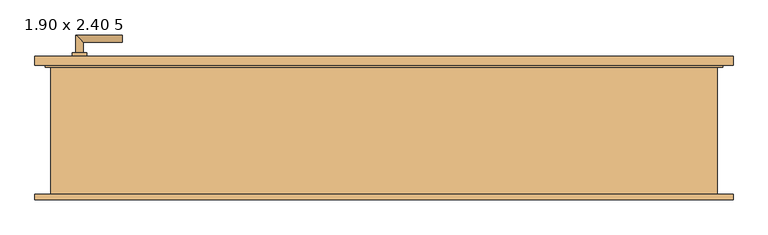
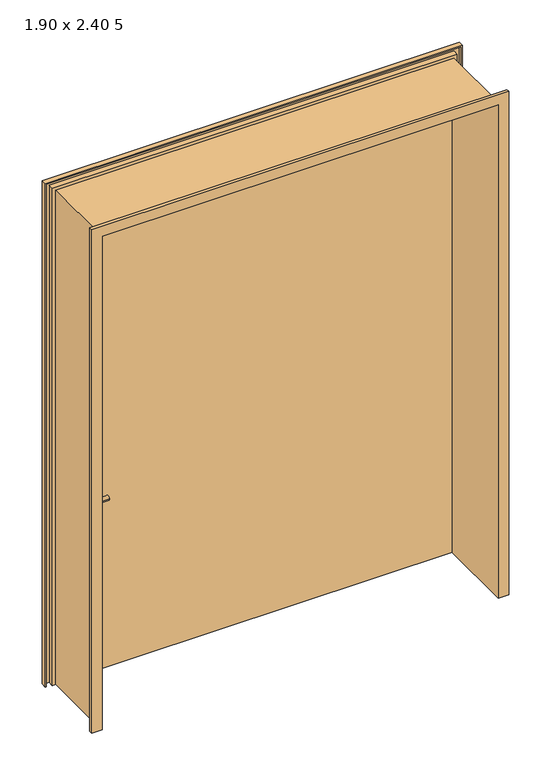
"""IFC4 building model written with IfcOpenShell, lengths in millimetres: door geometry, Drehflügel 1-flg - Stahlzarge : 1.90 x 2.40 5."""

from ifc_helpers import new_model, si_unit, point, frame, frame_2d, origin, place, context, project, spatial, polyline, circle_curve, ellipse_curve, trimmed, segment, composite_curve, outline, extrude, faceted_brep, source, transform, mapped, element, save
from ifc_brep_helpers import plane_surface, cylinder_surface, advanced_brep


def door_1_90_x_2_40_5_d04c458a(model_context):
    return source(origin(), model_context, "Body", "SolidModel", [
        advanced_brep(
        [(-860.0, 169.4346141, 1000.0), (-840.0, 169.4346141, 1000.0), (-860.0, 99.4346141, 1000.0), (-840.0, 119.4346141, 1000.0), (-730.0, 99.4346141, 1000.0), (-730.0, 119.4346141, 1000.0)],
        [
            (0, 1, circle_curve(frame((-850.0, 169.4346141, 1000.0), z_axis=(0.0, 1.0, 0.0), x_axis=(1.0, 0.0, 0.0)), 10.0)),
            (1, 0, circle_curve(frame((-850.0, 169.4346141, 1000.0), z_axis=(0.0, 1.0, 0.0), x_axis=(1.0, 0.0, 0.0)), 10.0)),
            (0, 2),
            (2, 3, ellipse_curve(frame((-850.0, 109.4346141, 1000.0), z_axis=(-0.7071067811865385, 0.7071067811865565, 0.0), x_axis=(0.7071067811865563, 0.7071067811865386, 0.0)), 14.1421356, 10.0)),
            (3, 1),
            (3, 2, ellipse_curve(frame((-850.0, 109.4346141, 1000.0), z_axis=(-0.7071067811865385, 0.7071067811865565, 0.0), x_axis=(0.7071067811865563, 0.7071067811865386, 0.0)), 14.1421356, 10.0)),
            (4, 5, circle_curve(frame((-730.0, 109.4346141, 1000.0), z_axis=(1.0, 0.0, 0.0), x_axis=(0.0, 1.0, 0.0)), 10.0)),
            (5, 4, circle_curve(frame((-730.0, 109.4346141, 1000.0), z_axis=(1.0, 0.0, 0.0), x_axis=(0.0, 1.0, 0.0)), 10.0)),
            (2, 4),
            (5, 3),
        ],
        [
            plane_surface(frame((-850.0, 169.4346141, -287.7526403), z_axis=(0.0, 1.0, 0.0), x_axis=(0.0, 0.0, 1.0))),
            cylinder_surface(frame((-850.0, 169.4346141, 1000.0), z_axis=(0.0, 1.0, 0.0), x_axis=(1.0, 0.0, 0.0)), 10.0),
            plane_surface(frame((-730.0, 109.4346141, -287.7526403), z_axis=(1.0, 0.0, 0.0), x_axis=(0.0, 0.0, 1.0))),
            cylinder_surface(frame((-850.0, 109.4346141, 1000.0), z_axis=(-1.0, 0.0, 0.0), x_axis=(0.0, 1.0, 0.0)), 10.0),
        ],
        [
            (0, [[1, 2]]),
            (1, [[-1, 3, 4, 5]]),
            (1, [[-2, -5, 6, -3]]),
            (2, [[7, 8]]),
            (3, [[-4, 9, -8, 10]]),
            (3, [[-6, -10, -7, -9]]),
        ],
    ),
        advanced_brep(
        [(-840.0, 229.4346141, 1000.0), (-860.0, 229.4346141, 1000.0), (-840.0, 259.4346141, 1000.0), (-860.0, 279.4346141, 1000.0), (-730.0, 259.4346141, 1000.0), (-730.0, 279.4346141, 1000.0)],
        [
            (0, 1, circle_curve(frame((-850.0, 229.4346141, 1000.0), z_axis=(0.0, -1.0, 0.0), x_axis=(-1.0, 0.0, 0.0)), 10.0)),
            (1, 0, circle_curve(frame((-850.0, 229.4346141, 1000.0), z_axis=(0.0, -1.0, 0.0), x_axis=(-1.0, 0.0, 0.0)), 10.0)),
            (0, 2),
            (2, 3, ellipse_curve(frame((-850.0, 269.4346141, 1000.0), z_axis=(-0.7071067811865475, -0.7071067811865475, 0.0), x_axis=(0.7071067811865474, -0.7071067811865476, 0.0)), 14.1421356, 10.0)),
            (3, 1),
            (3, 2, ellipse_curve(frame((-850.0, 269.4346141, 1000.0), z_axis=(-0.7071067811865475, -0.7071067811865475, 0.0), x_axis=(0.7071067811865474, -0.7071067811865476, 0.0)), 14.1421356, 10.0)),
            (4, 5, circle_curve(frame((-730.0, 269.4346141, 1000.0), z_axis=(1.0, 0.0, 0.0), x_axis=(0.0, 1.0, 0.0)), 10.0)),
            (5, 4, circle_curve(frame((-730.0, 269.4346141, 1000.0), z_axis=(1.0, 0.0, 0.0), x_axis=(0.0, 1.0, 0.0)), 10.0)),
            (2, 4),
            (5, 3),
        ],
        [
            plane_surface(frame((-850.0, 229.4346141, -287.7526403), z_axis=(0.0, -1.0, 0.0), x_axis=(0.0, 0.0, 1.0))),
            cylinder_surface(frame((-850.0, 229.4346141, 1000.0), z_axis=(0.0, -1.0, 0.0), x_axis=(-1.0, 0.0, 0.0)), 10.0),
            plane_surface(frame((-730.0, 269.4346141, -287.7526403), z_axis=(1.0, 0.0, 0.0), x_axis=(0.0, 0.0, 1.0))),
            cylinder_surface(frame((-850.0, 269.4346141, 1000.0), z_axis=(-1.0, 0.0, 0.0), x_axis=(0.0, 1.0, 0.0)), 10.0),
        ],
        [
            (0, [[1, 2]]),
            (1, [[-1, 3, 4, 5]]),
            (1, [[-2, -5, 6, -3]]),
            (2, [[7, 8]]),
            (3, [[-4, 9, -8, 10]]),
            (3, [[-6, -10, -7, -9]]),
        ],
    ),
        extrude(outline(composite_curve([segment(trimmed(circle_curve(frame_2d((1000.0, -850.0)), 20.0), [point((1000.0, -870.0))], [point((1000.0, -830.0))], False, "CARTESIAN"), True, "CONTINUOUS"), segment(trimmed(circle_curve(frame_2d((1000.0, -850.0)), 20.0), [point((1000.0, -830.0))], [point((1000.0, -870.0))], False, "CARTESIAN"), True, "CONTINUOUS")], self_intersect=False)), frame((0.0, 159.4346141, 0.0), z_axis=(0.0, 1.0, 0.0), x_axis=(0.0, 0.0, 1.0)), (0.0, 0.0, 1.0), 10.0),
        extrude(outline(composite_curve([segment(trimmed(circle_curve(frame_2d((1000.0, -850.0)), 20.0), [point((1000.0, -870.0))], [point((1000.0, -830.0))], False, "CARTESIAN"), True, "CONTINUOUS"), segment(trimmed(circle_curve(frame_2d((1000.0, -850.0)), 20.0), [point((1000.0, -830.0))], [point((1000.0, -870.0))], False, "CARTESIAN"), True, "CONTINUOUS")], self_intersect=False)), frame((0.0, 219.4346141, 0.0), z_axis=(0.0, 1.0, 0.0), x_axis=(0.0, 0.0, 1.0)), (0.0, 0.0, 1.0), 10.0),
        extrude(outline(polyline([(940.0, 194.4346141), (-940.0, 194.4346141), (-940.0, 219.4346141), (940.0, 219.4346141), (940.0, 194.4346141)])), frame((0.0, 0.0, 100.0), z_axis=(0.0, 0.0, 1.0), x_axis=(1.0, 0.0, 0.0)), (0.0, 0.0, 1.0), 2450.0),
        faceted_brep([(974.4603207, -180.5653859, 100.0), (925.0, -180.5653859, 100.0), (925.0, 194.4346141, 100.0), (940.0, 194.4346141, 100.0), (940.0, 219.4346141, 100.0), (974.4603207, 219.4346141, 100.0), (974.4603207, 194.4346141, 100.0), (969.4603207, 194.4346141, 100.0), (969.4603207, 214.4346141, 100.0), (945.0, 214.4346141, 100.0), (945.0, 189.4346141, 100.0), (930.0, 189.4346141, 100.0), (930.0, -175.5653859, 100.0), (969.4603207, -175.5653859, 100.0), (969.4603207, -165.5653859, 100.0), (974.4603207, -165.5653859, 100.0), (974.4603207, -180.5653859, 2584.4603207), (-974.4603207, -180.5653859, 2584.4603207), (-974.4603207, -180.5653859, 100.0), (-925.0, -180.5653859, 100.0), (-925.0, -180.5653859, 2535.0), (925.0, -180.5653859, 2535.0), (925.0, 194.4346141, 2535.0), (-925.0, 194.4346141, 2535.0), (-925.0, 194.4346141, 100.0), (-940.0, 194.4346141, 100.0), (-940.0, 194.4346141, 2550.0), (940.0, 194.4346141, 2550.0), (940.0, 219.4346141, 2550.0), (-940.0, 219.4346141, 2550.0), (-940.0, 219.4346141, 100.0), (-974.4603207, 219.4346141, 100.0), (-974.4603207, 219.4346141, 2584.4603207), (974.4603207, 219.4346141, 2584.4603207), (974.4603207, 194.4346141, 2584.4603207), (-974.4603207, 194.4346141, 2584.4603207), (-974.4603207, 194.4346141, 100.0), (-969.4603207, 194.4346141, 100.0), (-969.4603207, 194.4346141, 2579.4603207), (969.4603207, 194.4346141, 2579.4603207), (969.4603207, 214.4346141, 2579.4603207), (-969.4603207, 214.4346141, 2579.4603207), (-969.4603207, 214.4346141, 100.0), (-945.0, 214.4346141, 100.0), (-945.0, 214.4346141, 2555.0), (945.0, 214.4346141, 2555.0), (945.0, 189.4346141, 2555.0), (-945.0, 189.4346141, 2555.0), (-945.0, 189.4346141, 100.0), (-930.0, 189.4346141, 100.0), (-930.0, 189.4346141, 2540.0), (930.0, 189.4346141, 2540.0), (930.0, -175.5653859, 2540.0), (-930.0, -175.5653859, 2540.0), (-930.0, -175.5653859, 100.0), (-969.4603207, -175.5653859, 100.0), (-969.4603207, -175.5653859, 2579.4603207), (969.4603207, -175.5653859, 2579.4603207), (969.4603207, -165.5653859, 2579.4603207), (-969.4603207, -165.5653859, 2579.4603207), (-969.4603207, -165.5653859, 100.0), (-974.4603207, -165.5653859, 100.0), (-974.4603207, -165.5653859, 2584.4603207), (974.4603207, -165.5653859, 2584.4603207)], [[[0, 1, 2, 3, 4, 5, 6, 7, 8, 9, 10, 11, 12, 13, 14, 15]], [[1, 0, 16, 17, 18, 19, 20, 21]], [[2, 1, 21, 22]], [[3, 2, 22, 23, 24, 25, 26, 27]], [[4, 3, 27, 28]], [[5, 4, 28, 29, 30, 31, 32, 33]], [[6, 5, 33, 34]], [[7, 6, 34, 35, 36, 37, 38, 39]], [[8, 7, 39, 40]], [[9, 8, 40, 41, 42, 43, 44, 45]], [[10, 9, 45, 46]], [[11, 10, 46, 47, 48, 49, 50, 51]], [[12, 11, 51, 52]], [[13, 12, 52, 53, 54, 55, 56, 57]], [[14, 13, 57, 58]], [[15, 14, 58, 59, 60, 61, 62, 63]], [[0, 15, 63, 16]], [[17, 62, 61, 18]], [[18, 61, 60, 55, 54, 49, 48, 43, 42, 37, 36, 31, 30, 25, 24, 19]], [[23, 20, 19, 24]], [[29, 26, 25, 30]], [[35, 32, 31, 36]], [[41, 38, 37, 42]], [[47, 44, 43, 48]], [[53, 50, 49, 54]], [[59, 56, 55, 60]], [[22, 21, 20, 23]], [[28, 27, 26, 29]], [[34, 33, 32, 35]], [[40, 39, 38, 41]], [[46, 45, 44, 47]], [[52, 51, 50, 53]], [[58, 57, 56, 59]], [[16, 63, 62, 17]]]),
    ])


if __name__ == "__main__":
    model = new_model("IFC4")
    model_context = context("Model", 3, world=origin())
    ifc_project = project(units=[si_unit("LENGTHUNIT", "METRE", prefix="MILLI")], contexts=[model_context])
    site = spatial("IfcSite", under=ifc_project)
    building = spatial("IfcBuilding", under=site)
    placement = place(None, origin())
    door_1_90_x_2_40_5_shape = door_1_90_x_2_40_5_d04c458a(model_context)
    element("IfcDoor", 1, ObjectType="Drehflügel 1-flg - Stahlzarge : 1.90 x 2.40 5", at=placement, inside=building, context=model_context, shape_type="MappedRepresentation", body=[
        mapped(door_1_90_x_2_40_5_shape, transform((0.0, 0.0, 0.0), x_axis=(1.0, 0.0, 0.0), y_axis=(0.0, 1.0, 0.0), z_axis=(0.0, 0.0, 1.0))),
    ])
    save(model, "model.ifc")

# Revit data of these elements
# Type "Drehflügel 1-flg - Stahlzarge : 1.90 x 2.40 5"
#   Type Mark = "27"
#   Operation = "SingleSwingRight"
#   Keynote = "16.03"
#   Analytic Construction = "Metall"
#   Thermal Resistance (R) = 0.270117 (m²·K)/W
#   Heat Transfer Coefficient (U) = 3.7021 W/(m²·K)
#   Rough Width = 1.900 m
#   Rough Height [instance default] = 2.560 m
#   Höhe Türgriff [instance default] = 0.900 m
#   Height = 2.460 m
#   Fußbodenaufbau [instance default] = 0.100 m
#   Width = 1.900 m
#   Sichtbarkeit Sturzlinien [instance default] = yes
#   Türgriff auswählen [instance default] = element 221079
#   Türgriff [instance default] = none
#   Türflügel [instance default] = none
#   Rahmen/Pfosten [instance default] = Metall - Lackiert - Grau
#   Visual Light Transmittance = 0
#   Solar Heat Gain Coefficient = 0
#   Function = (empty or 0)
#   Wall Closure = (empty or 0)
# Element 1 (IfcDoor, "Drehflügel 1-flg - Stahlzarge : 1.90 x 2.40 5")
#   Materials on its faces: "Metall - Lackiert - Grau", "Metall - Chrom", "Holz - Birke"
# Materials
#   "Metall - Lackiert - Grau": class "Farbe 1", colour RGB 98 98 98, transparency 0, Cost = 0
#   "Metall - Chrom": class "Metall", colour RGB 247 247 247, transparency 0, Cost = 0
#   "Holz - Birke": class "Holz", colour RGB 213 164 103, transparency 0, Cost = 0
